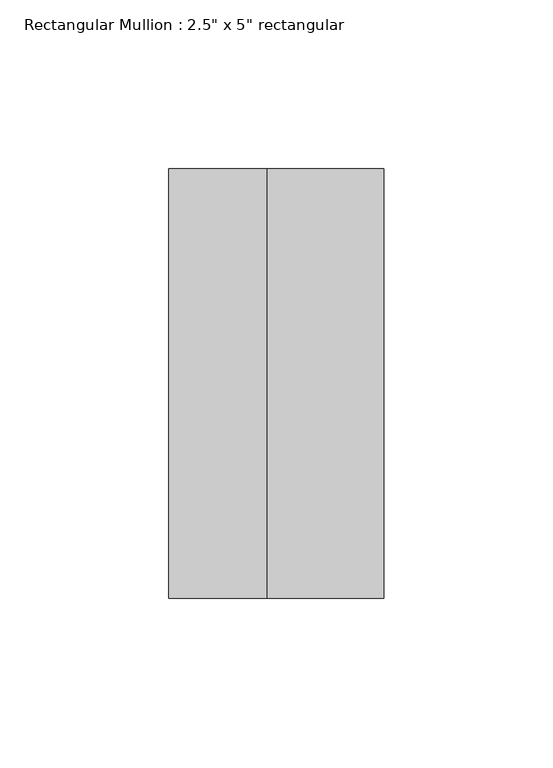
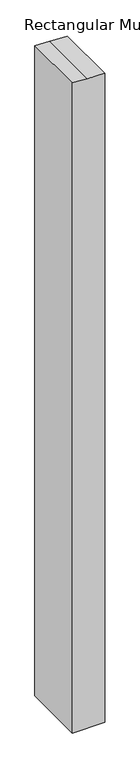
"""IFC4 building model written with IfcOpenShell, lengths in millimetres: member geometry."""

import ifcopenshell
import ifcopenshell.guid

model = None  # the IFC model being written
_history = None  # IfcOwnerHistory: only IFC2X3 demands one
_inside = {}  # id of a spatial element -> (the spatial element, [elements in it])
_under = {}  # id of a project, library or spatial element -> (it, [spatial elements below it])
_declared = {}  # id of a project -> (the project, [libraries it declares])
_typed = {}  # id of a type object -> (the type object, [elements of that type])
_made_of = {}  # id of a material, layer set ... -> (it, [elements and type objects made of it])


def new_model(schema):
    """Start an empty IFC model of exactly this schema.

    Asked for "IFC4X3", IfcOpenShell would pick the latest addendum, in which some entities
    have other attributes; the version numbers below select the first issue.
    IFC2X3 requires an IfcOwnerHistory on every rooted entity: one is made here for all.
    """
    global model, _history
    if schema == "IFC4X3":
        model = ifcopenshell.file(schema_version=(4, 3, 0, 0))
    else:
        model = ifcopenshell.file(schema=schema)
    _inside.clear()
    _under.clear()
    _declared.clear()
    _typed.clear()
    _made_of.clear()
    _history = None
    if model.schema == "IFC2X3":
        org = make("IfcOrganization", Name="unknown")
        user = make(
            "IfcPersonAndOrganization",
            ThePerson=make("IfcPerson", FamilyName="unknown"),
            TheOrganization=org,
        )
        app = make(
            "IfcApplication",
            ApplicationDeveloper=org,
            Version="unknown",
            ApplicationFullName="unknown",
            ApplicationIdentifier="unknown",
        )
        _history = make(
            "IfcOwnerHistory",
            OwningUser=user,
            OwningApplication=app,
            ChangeAction="ADDED",
            CreationDate=0,
        )
    return model


def make(cls, **values):
    """One entity of the class cls with the attributes given. An attribute that is None is left unset."""
    return model.create_entity(
        cls, **{name: value for name, value in values.items() if value is not None}
    )


def rooted(cls, **values):
    """An entity with a GlobalId (a new one), such as an element, a storey or a relation."""
    return make(cls, GlobalId=ifcopenshell.guid.new(), OwnerHistory=_history, **values)


def si_unit(unit_type, name, prefix=None):
    """IfcSIUnit, for example si_unit("LENGTHUNIT", "METRE", prefix="MILLI")."""
    return make("IfcSIUnit", UnitType=unit_type, Prefix=prefix, Name=name)


def assignment(units):
    """IfcUnitAssignment: the units of a project."""
    return None if units is None else make("IfcUnitAssignment", Units=units)


def point(xyz):
    """IfcCartesianPoint."""
    return None if xyz is None else make("IfcCartesianPoint", Coordinates=xyz)


def direction(xyz):
    """IfcDirection."""
    return None if xyz is None else make("IfcDirection", DirectionRatios=xyz)


def frame(location, z_axis=None, x_axis=None):
    """IfcAxis2Placement3D, a coordinate frame: its origin and axes. An axis left out is left unset."""
    return make(
        "IfcAxis2Placement3D",
        Location=point(location),
        Axis=direction(z_axis),
        RefDirection=direction(x_axis),
    )


def origin():
    """The frame at (0, 0, 0) with its axes left unset."""
    return frame((0.0, 0.0, 0.0))


def place(relative_to, where):
    """IfcLocalPlacement: puts the frame where relative to a parent placement (None: the world)."""
    return make(
        "IfcLocalPlacement", PlacementRelTo=relative_to, RelativePlacement=where
    )


def context(
    kind, dimensions, precision=None, world=None, true_north=None, identifier=None
):
    """IfcGeometricRepresentationContext, for example the 3D "Model" context."""
    return make(
        "IfcGeometricRepresentationContext",
        ContextIdentifier=identifier,
        ContextType=kind,
        CoordinateSpaceDimension=dimensions,
        Precision=precision,
        WorldCoordinateSystem=world,
        TrueNorth=true_north,
    )


def project(units=None, contexts=None):
    """IfcProject with its units and contexts."""
    return rooted(
        "IfcProject",
        Name="project",
        RepresentationContexts=contexts,
        UnitsInContext=assignment(units),
    )


def spatial(cls, under=None, at=None, **own):
    """A site, building, storey or space (cls), placed at a placement, below another one or the project."""
    s = rooted(cls, ObjectPlacement=at, **own)
    if under is not None:
        _under.setdefault(under.id(), (under, []))[1].append(s)
    return s


def polyline(points):
    """IfcPolyline through the points."""
    return make("IfcPolyline", Points=[point(p) for p in points])


def outline(outer, holes=None, kind="AREA"):
    """IfcArbitraryClosedProfileDef: a profile drawn as a closed curve; with holes, ...WithVoids."""
    if holes is None:
        return make("IfcArbitraryClosedProfileDef", ProfileType=kind, OuterCurve=outer)
    return make(
        "IfcArbitraryProfileDefWithVoids",
        ProfileType=kind,
        OuterCurve=outer,
        InnerCurves=holes,
    )


def extrude(swept, where, along, depth):
    """IfcExtrudedAreaSolid: the profile swept, set in the frame where, extruded along a direction by depth."""
    return make(
        "IfcExtrudedAreaSolid",
        SweptArea=swept,
        Position=where,
        ExtrudedDirection=direction(along),
        Depth=depth,
    )


def shape(context_of_items, identifier, shape_type, items):
    """IfcShapeRepresentation: the items that make up one representation, for example the "Body"."""
    return make(
        "IfcShapeRepresentation",
        ContextOfItems=context_of_items,
        RepresentationIdentifier=identifier,
        RepresentationType=shape_type,
        Items=items,
    )


def source(mapping_origin, context_of_items, identifier, shape_type, items):
    """IfcRepresentationMap: a shape defined once, which mapped items show again and again."""
    return make(
        "IfcRepresentationMap",
        MappingOrigin=mapping_origin,
        MappedRepresentation=shape(context_of_items, identifier, shape_type, items),
    )


def transform(
    local_origin,
    x_axis=None,
    y_axis=None,
    z_axis=None,
    scale=None,
    scale2=None,
    scale3=None,
    uniform=True,
):
    """IfcCartesianTransformationOperator3D, or its non-uniform kind. x_axis, y_axis, z_axis: its Axis1, 2, 3."""
    if uniform:
        return make(
            "IfcCartesianTransformationOperator3D",
            Axis1=direction(x_axis),
            Axis2=direction(y_axis),
            LocalOrigin=point(local_origin),
            Scale=scale,
            Axis3=direction(z_axis),
        )
    return make(
        "IfcCartesianTransformationOperator3DnonUniform",
        Axis1=direction(x_axis),
        Axis2=direction(y_axis),
        LocalOrigin=point(local_origin),
        Scale=scale,
        Axis3=direction(z_axis),
        Scale2=scale2,
        Scale3=scale3,
    )


def mapped(mapping_source, mapping_target):
    """IfcMappedItem: shows the shape of a source again, moved by a transform."""
    return make(
        "IfcMappedItem", MappingSource=mapping_source, MappingTarget=mapping_target
    )


def made_of(thing, what):
    """Note that an element or type object is made of a material, layer set ...; save() writes the relation."""
    if what is not None:
        _made_of.setdefault(what.id(), (what, []))[1].append(thing)
    return thing


def element(
    cls,
    number,
    at=None,
    inside=None,
    cuts=None,
    type_object=None,
    material=None,
    context=None,
    identifier="Body",
    shape_type=None,
    held_by="IfcProductDefinitionShape",
    body=None,
    shapes=None,
    **own,
):
    """One element of the class cls, such as IfcWall. Its Tag is "e" and its number.

    at: its placement. inside: the storey or other place that contains it. cuts: it is an
    opening in that element (IfcRelVoidsElement). A single representation is given by context,
    identifier, shape_type and body (its items); several are given by shapes. held_by: the class
    of the entity that holds the representations. save() writes the other relations.
    """
    e = rooted(cls, Tag="e%d" % number, ObjectPlacement=at, **own)
    if body is not None:
        shapes = [shape(context, identifier, shape_type, body)]
    if shapes is not None:
        e.Representation = make(held_by, Representations=shapes)
    if inside is not None:
        _inside.setdefault(inside.id(), (inside, []))[1].append(e)
    if cuts is not None:
        rooted(
            "IfcRelVoidsElement", RelatingBuildingElement=cuts, RelatedOpeningElement=e
        )
    if type_object is not None:
        _typed.setdefault(type_object.id(), (type_object, []))[1].append(e)
    return made_of(e, material)


def aggregate(whole, parts):
    """IfcRelAggregates: a whole, such as a stair, and the parts it consists of."""
    return rooted("IfcRelAggregates", RelatingObject=whole, RelatedObjects=parts)


def save(model, path):
    """Write the relations noted so far, then the file.

    IfcRelAggregates (storeys below a building ...), IfcRelContainedInSpatialStructure (elements
    in a storey), IfcRelDefinesByType, IfcRelAssociatesMaterial and IfcRelDeclares: one each for
    every whole, place, type object, material and project.
    """
    for whole, parts in _under.values():
        aggregate(whole, parts)
    for where, things in _inside.values():
        rooted(
            "IfcRelContainedInSpatialStructure",
            RelatedElements=things,
            RelatingStructure=where,
        )
    for kind, things in _typed.values():
        rooted("IfcRelDefinesByType", RelatedObjects=things, RelatingType=kind)
    for what, things in _made_of.values():
        rooted("IfcRelAssociatesMaterial", RelatedObjects=things, RelatingMaterial=what)
    for by, libraries in _declared.values():
        rooted("IfcRelDeclares", RelatingContext=by, RelatedDefinitions=libraries)
    model.write(path)


def member_9d221ad8(model_context):
    return source(origin(), model_context, "Body", "SweptSolid", [
        extrude(outline(polyline([(-64.8775557, 31.75), (-63.4449853, -2.6426951), (-62.232569, -31.75), (-1407.9643899, -31.75), (-1407.9643899, 31.75), (-64.8775557, 31.75)])), frame((0.0, -63.5, 0.0), z_axis=(0.0, 1.0, 0.0), x_axis=(0.0, 0.0, 1.0)), (0.0, 0.0, 1.0), 127.0),
    ])


if __name__ == "__main__":
    model = new_model("IFC4")
    model_context = context("Model", 3, world=origin())
    ifc_project = project(units=[si_unit("LENGTHUNIT", "METRE", prefix="MILLI")], contexts=[model_context])
    site = spatial("IfcSite", under=ifc_project)
    building = spatial("IfcBuilding", under=site)
    placement = place(None, origin())
    member_shape = member_9d221ad8(model_context)
    element("IfcMember", 1, ObjectType="Rectangular Mullion : 2.5\" x 5\" rectangular", at=placement, inside=building, context=model_context, shape_type="MappedRepresentation", body=[
        mapped(member_shape, transform((0.0, 0.0, 0.0), x_axis=(1.0, 0.0, 0.0), y_axis=(0.0, 1.0, 0.0), z_axis=(0.0, 0.0, 1.0))),
    ])
    save(model, "model.ifc")

# Revit data of these elements
# Type "Rectangular Mullion : 2.5\" x 5\" rectangular"
#   built-in parameter 1007304 = 0.416667 (stored number, unit not read)
#   built-in parameter 1007301 = 0.104167 (stored number, unit not read)
#   built-in parameter 1007300 = 0.104167 (stored number, unit not read)
# Element 1 (IfcMember, "Rectangular Mullion : 2.5\" x 5\" rectangular")
#   Materials on its faces: "Aluminum"
# Materials
#   "Aluminum": class "Metal", colour RGB 247 247 247, transparency 0, Description = "Aluminum 6061", Cost = 0
